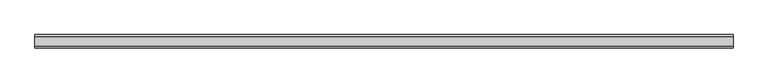
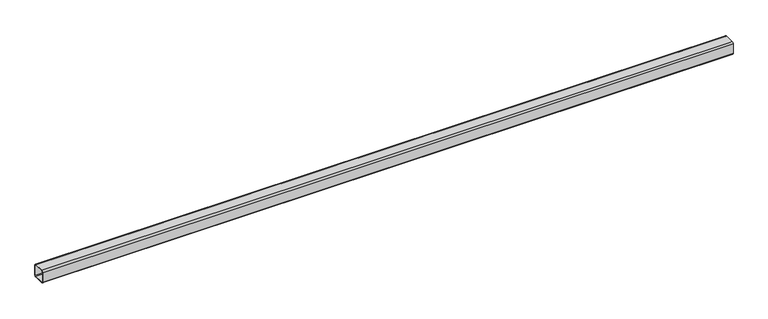
"""IFC4 building model written with IfcOpenShell, lengths in millimetres: beam geometry, Гнутый прямоугольный профиль (Трубы 30245-94) Балки : гнутый прямоуг. проф. 100x6."""

import ifcopenshell
import ifcopenshell.guid

model = None  # the IFC model being written
_history = None  # IfcOwnerHistory: only IFC2X3 demands one
_inside = {}  # id of a spatial element -> (the spatial element, [elements in it])
_under = {}  # id of a project, library or spatial element -> (it, [spatial elements below it])
_declared = {}  # id of a project -> (the project, [libraries it declares])
_typed = {}  # id of a type object -> (the type object, [elements of that type])
_made_of = {}  # id of a material, layer set ... -> (it, [elements and type objects made of it])


def new_model(schema):
    """Start an empty IFC model of exactly this schema.

    Asked for "IFC4X3", IfcOpenShell would pick the latest addendum, in which some entities
    have other attributes; the version numbers below select the first issue.
    IFC2X3 requires an IfcOwnerHistory on every rooted entity: one is made here for all.
    """
    global model, _history
    if schema == "IFC4X3":
        model = ifcopenshell.file(schema_version=(4, 3, 0, 0))
    else:
        model = ifcopenshell.file(schema=schema)
    _inside.clear()
    _under.clear()
    _declared.clear()
    _typed.clear()
    _made_of.clear()
    _history = None
    if model.schema == "IFC2X3":
        org = make("IfcOrganization", Name="unknown")
        user = make(
            "IfcPersonAndOrganization",
            ThePerson=make("IfcPerson", FamilyName="unknown"),
            TheOrganization=org,
        )
        app = make(
            "IfcApplication",
            ApplicationDeveloper=org,
            Version="unknown",
            ApplicationFullName="unknown",
            ApplicationIdentifier="unknown",
        )
        _history = make(
            "IfcOwnerHistory",
            OwningUser=user,
            OwningApplication=app,
            ChangeAction="ADDED",
            CreationDate=0,
        )
    return model


def make(cls, **values):
    """One entity of the class cls with the attributes given. An attribute that is None is left unset."""
    return model.create_entity(
        cls, **{name: value for name, value in values.items() if value is not None}
    )


def rooted(cls, **values):
    """An entity with a GlobalId (a new one), such as an element, a storey or a relation."""
    return make(cls, GlobalId=ifcopenshell.guid.new(), OwnerHistory=_history, **values)


def si_unit(unit_type, name, prefix=None):
    """IfcSIUnit, for example si_unit("LENGTHUNIT", "METRE", prefix="MILLI")."""
    return make("IfcSIUnit", UnitType=unit_type, Prefix=prefix, Name=name)


def assignment(units):
    """IfcUnitAssignment: the units of a project."""
    return None if units is None else make("IfcUnitAssignment", Units=units)


def point(xyz):
    """IfcCartesianPoint."""
    return None if xyz is None else make("IfcCartesianPoint", Coordinates=xyz)


def direction(xyz):
    """IfcDirection."""
    return None if xyz is None else make("IfcDirection", DirectionRatios=xyz)


def frame(location, z_axis=None, x_axis=None):
    """IfcAxis2Placement3D, a coordinate frame: its origin and axes. An axis left out is left unset."""
    return make(
        "IfcAxis2Placement3D",
        Location=point(location),
        Axis=direction(z_axis),
        RefDirection=direction(x_axis),
    )


def frame_2d(location, x_axis=None):
    """IfcAxis2Placement2D, a coordinate frame in the plane: its origin and x axis."""
    return make(
        "IfcAxis2Placement2D", Location=point(location), RefDirection=direction(x_axis)
    )


def origin():
    """The frame at (0, 0, 0) with its axes left unset."""
    return frame((0.0, 0.0, 0.0))


def place(relative_to, where):
    """IfcLocalPlacement: puts the frame where relative to a parent placement (None: the world)."""
    return make(
        "IfcLocalPlacement", PlacementRelTo=relative_to, RelativePlacement=where
    )


def context(
    kind, dimensions, precision=None, world=None, true_north=None, identifier=None
):
    """IfcGeometricRepresentationContext, for example the 3D "Model" context."""
    return make(
        "IfcGeometricRepresentationContext",
        ContextIdentifier=identifier,
        ContextType=kind,
        CoordinateSpaceDimension=dimensions,
        Precision=precision,
        WorldCoordinateSystem=world,
        TrueNorth=true_north,
    )


def project(units=None, contexts=None):
    """IfcProject with its units and contexts."""
    return rooted(
        "IfcProject",
        Name="project",
        RepresentationContexts=contexts,
        UnitsInContext=assignment(units),
    )


def spatial(cls, under=None, at=None, **own):
    """A site, building, storey or space (cls), placed at a placement, below another one or the project."""
    s = rooted(cls, ObjectPlacement=at, **own)
    if under is not None:
        _under.setdefault(under.id(), (under, []))[1].append(s)
    return s


def polyline(points):
    """IfcPolyline through the points."""
    return make("IfcPolyline", Points=[point(p) for p in points])


def circle_curve(where, radius):
    """IfcCircle in the frame where."""
    return make("IfcCircle", Position=where, Radius=radius)


def trimmed(basis, trim1, trim2, sense, master):
    """IfcTrimmedCurve: the piece of a basis curve between two trims."""
    return make(
        "IfcTrimmedCurve",
        BasisCurve=basis,
        Trim1=trim1,
        Trim2=trim2,
        SenseAgreement=sense,
        MasterRepresentation=master,
    )


def segment(curve, same_sense, transition):
    """IfcCompositeCurveSegment."""
    return make(
        "IfcCompositeCurveSegment",
        Transition=transition,
        SameSense=same_sense,
        ParentCurve=curve,
    )


def composite_curve(segments, self_intersect=None):
    """IfcCompositeCurve: segments joined end to end."""
    return make("IfcCompositeCurve", Segments=segments, SelfIntersect=self_intersect)


def outline(outer, holes=None, kind="AREA"):
    """IfcArbitraryClosedProfileDef: a profile drawn as a closed curve; with holes, ...WithVoids."""
    if holes is None:
        return make("IfcArbitraryClosedProfileDef", ProfileType=kind, OuterCurve=outer)
    return make(
        "IfcArbitraryProfileDefWithVoids",
        ProfileType=kind,
        OuterCurve=outer,
        InnerCurves=holes,
    )


def extrude(swept, where, along, depth):
    """IfcExtrudedAreaSolid: the profile swept, set in the frame where, extruded along a direction by depth."""
    return make(
        "IfcExtrudedAreaSolid",
        SweptArea=swept,
        Position=where,
        ExtrudedDirection=direction(along),
        Depth=depth,
    )


def shape(context_of_items, identifier, shape_type, items):
    """IfcShapeRepresentation: the items that make up one representation, for example the "Body"."""
    return make(
        "IfcShapeRepresentation",
        ContextOfItems=context_of_items,
        RepresentationIdentifier=identifier,
        RepresentationType=shape_type,
        Items=items,
    )


def source(mapping_origin, context_of_items, identifier, shape_type, items):
    """IfcRepresentationMap: a shape defined once, which mapped items show again and again."""
    return make(
        "IfcRepresentationMap",
        MappingOrigin=mapping_origin,
        MappedRepresentation=shape(context_of_items, identifier, shape_type, items),
    )


def transform(
    local_origin,
    x_axis=None,
    y_axis=None,
    z_axis=None,
    scale=None,
    scale2=None,
    scale3=None,
    uniform=True,
):
    """IfcCartesianTransformationOperator3D, or its non-uniform kind. x_axis, y_axis, z_axis: its Axis1, 2, 3."""
    if uniform:
        return make(
            "IfcCartesianTransformationOperator3D",
            Axis1=direction(x_axis),
            Axis2=direction(y_axis),
            LocalOrigin=point(local_origin),
            Scale=scale,
            Axis3=direction(z_axis),
        )
    return make(
        "IfcCartesianTransformationOperator3DnonUniform",
        Axis1=direction(x_axis),
        Axis2=direction(y_axis),
        LocalOrigin=point(local_origin),
        Scale=scale,
        Axis3=direction(z_axis),
        Scale2=scale2,
        Scale3=scale3,
    )


def mapped(mapping_source, mapping_target):
    """IfcMappedItem: shows the shape of a source again, moved by a transform."""
    return make(
        "IfcMappedItem", MappingSource=mapping_source, MappingTarget=mapping_target
    )


def made_of(thing, what):
    """Note that an element or type object is made of a material, layer set ...; save() writes the relation."""
    if what is not None:
        _made_of.setdefault(what.id(), (what, []))[1].append(thing)
    return thing


def element(
    cls,
    number,
    at=None,
    inside=None,
    cuts=None,
    type_object=None,
    material=None,
    context=None,
    identifier="Body",
    shape_type=None,
    held_by="IfcProductDefinitionShape",
    body=None,
    shapes=None,
    **own,
):
    """One element of the class cls, such as IfcWall. Its Tag is "e" and its number.

    at: its placement. inside: the storey or other place that contains it. cuts: it is an
    opening in that element (IfcRelVoidsElement). A single representation is given by context,
    identifier, shape_type and body (its items); several are given by shapes. held_by: the class
    of the entity that holds the representations. save() writes the other relations.
    """
    e = rooted(cls, Tag="e%d" % number, ObjectPlacement=at, **own)
    if body is not None:
        shapes = [shape(context, identifier, shape_type, body)]
    if shapes is not None:
        e.Representation = make(held_by, Representations=shapes)
    if inside is not None:
        _inside.setdefault(inside.id(), (inside, []))[1].append(e)
    if cuts is not None:
        rooted(
            "IfcRelVoidsElement", RelatingBuildingElement=cuts, RelatedOpeningElement=e
        )
    if type_object is not None:
        _typed.setdefault(type_object.id(), (type_object, []))[1].append(e)
    return made_of(e, material)


def aggregate(whole, parts):
    """IfcRelAggregates: a whole, such as a stair, and the parts it consists of."""
    return rooted("IfcRelAggregates", RelatingObject=whole, RelatedObjects=parts)


def save(model, path):
    """Write the relations noted so far, then the file.

    IfcRelAggregates (storeys below a building ...), IfcRelContainedInSpatialStructure (elements
    in a storey), IfcRelDefinesByType, IfcRelAssociatesMaterial and IfcRelDeclares: one each for
    every whole, place, type object, material and project.
    """
    for whole, parts in _under.values():
        aggregate(whole, parts)
    for where, things in _inside.values():
        rooted(
            "IfcRelContainedInSpatialStructure",
            RelatedElements=things,
            RelatingStructure=where,
        )
    for kind, things in _typed.values():
        rooted("IfcRelDefinesByType", RelatedObjects=things, RelatingType=kind)
    for what, things in _made_of.values():
        rooted("IfcRelAssociatesMaterial", RelatedObjects=things, RelatingMaterial=what)
    for by, libraries in _declared.values():
        rooted("IfcRelDeclares", RelatingContext=by, RelatedDefinitions=libraries)
    model.write(path)


def beam_6aa5ee4f(model_context):
    return source(origin(), model_context, "Body", "SweptSolid", [
        extrude(outline(composite_curve([segment(polyline([(-38.0, 50.0), (38.0, 50.0)]), True, "CONTINUOUS"), segment(trimmed(circle_curve(frame_2d((38.0, 38.0)), 12.0), [point((38.0, 50.0))], [point((50.0, 38.0))], False, "CARTESIAN"), True, "CONTINUOUS"), segment(polyline([(50.0, 38.0), (50.0, -38.0)]), True, "CONTINUOUS"), segment(trimmed(circle_curve(frame_2d((38.0, -38.0)), 12.0), [point((50.0, -38.0))], [point((38.0, -50.0))], False, "CARTESIAN"), True, "CONTINUOUS"), segment(polyline([(38.0, -50.0), (-38.0, -50.0)]), True, "CONTINUOUS"), segment(trimmed(circle_curve(frame_2d((-38.0, -38.0)), 12.0), [point((-38.0, -50.0))], [point((-50.0, -38.0))], False, "CARTESIAN"), True, "CONTINUOUS"), segment(polyline([(-50.0, -38.0), (-50.0, 38.0)]), True, "CONTINUOUS"), segment(trimmed(circle_curve(frame_2d((-38.0, 38.0)), 12.0), [point((-50.0, 38.0))], [point((-38.0, 50.0))], False, "CARTESIAN"), True, "CONTINUOUS")], self_intersect=False), holes=[composite_curve([segment(trimmed(circle_curve(frame_2d((-38.0, 38.0)), 6.0), [point((-38.0, 44.0))], [point((-44.0, 38.0))], True, "CARTESIAN"), True, "CONTINUOUS"), segment(polyline([(-44.0, 38.0), (-44.0, -38.0)]), True, "CONTINUOUS"), segment(trimmed(circle_curve(frame_2d((-38.0, -38.0)), 6.0), [point((-44.0, -38.0))], [point((-38.0, -44.0))], True, "CARTESIAN"), True, "CONTINUOUS"), segment(polyline([(-38.0, -44.0), (38.0, -44.0)]), True, "CONTINUOUS"), segment(trimmed(circle_curve(frame_2d((38.0, -38.0)), 6.0), [point((38.0, -44.0))], [point((44.0, -38.0))], True, "CARTESIAN"), True, "CONTINUOUS"), segment(polyline([(44.0, -38.0), (44.0, 38.0)]), True, "CONTINUOUS"), segment(trimmed(circle_curve(frame_2d((38.0, 38.0)), 6.0), [point((44.0, 38.0))], [point((38.0, 44.0))], True, "CARTESIAN"), True, "CONTINUOUS"), segment(polyline([(38.0, 44.0), (-38.0, 44.0)]), True, "CONTINUOUS")], self_intersect=False)]), frame((-2618.5, 0.0, 0.0), z_axis=(1.0, 0.0, 0.0), x_axis=(0.0, 1.0, 0.0)), (0.0, 0.0, 1.0), 5237.0),
    ])


if __name__ == "__main__":
    model = new_model("IFC4")
    model_context = context("Model", 3, world=origin())
    ifc_project = project(units=[si_unit("LENGTHUNIT", "METRE", prefix="MILLI")], contexts=[model_context])
    site = spatial("IfcSite", under=ifc_project)
    building = spatial("IfcBuilding", under=site)
    placement = place(None, origin())
    beam_shape = beam_6aa5ee4f(model_context)
    element("IfcBeam", 1, ObjectType="Гнутый прямоугольный профиль (Трубы 30245-94) Балки : гнутый прямоуг. проф. 100x6", at=placement, inside=building, context=model_context, shape_type="MappedRepresentation", body=[
        mapped(beam_shape, transform((0.0, 0.0, 0.0), x_axis=(1.0, 0.0, 0.0), y_axis=(0.0, 1.0, 0.0), z_axis=(0.0, 0.0, 1.0))),
    ])
    save(model, "model.ifc")

# Revit data of these elements
# Type "Гнутый прямоугольный профиль (Трубы 30245-94) Балки : гнутый прямоуг. проф. 100x6"
#   ri = 12 mm
#   ra = 6 mm
#   W = 0.173578
#   Vz = 50 mm
#   Vy = 50 mm
#   Vpz = 50 mm
#   Vpy = 50 mm
#   Length [instance default] = 1500 mm
#   bf = 100 mm
#   d = 100 mm
#   tf = 6 mm
#   tw = 6 mm
#   A = 0.00226 m²
#   Structural Material [instance default] = Металл - Сталь - 345 МПa
#   Assembly Code = ""
# Element 1 (IfcBeam, "Гнутый прямоугольный профиль (Трубы 30245-94) Балки : гнутый прямоуг. проф. 100x6")
#   Structural Material = C235
#   Materials on its faces: "C235"
# Materials
#   "Металл - Сталь - 345 МПa": class "Металл", colour RGB 247 247 247, transparency 0
#   "C235": class "Не назначено", colour RGB 0 0 0, transparency 0
